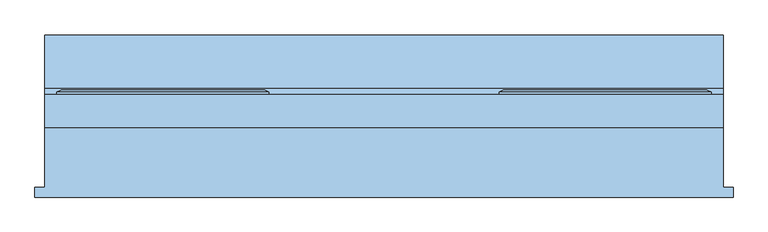
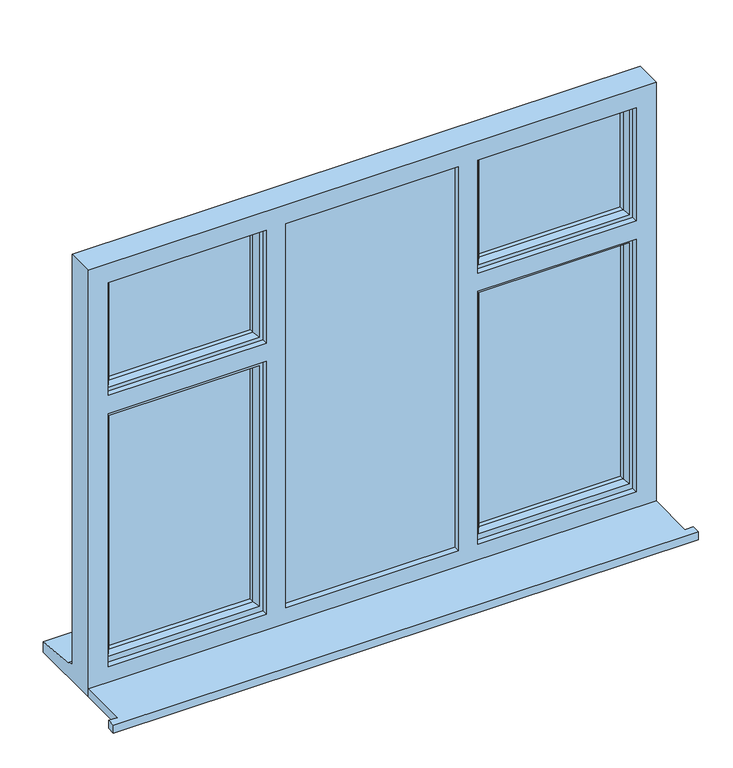
"""IFC4 building model written with IfcOpenShell, lengths in millimetres: window geometry, Window - Triple Casement with Top and Side Sashes : Window - Triple Casement with Top and Side Sashes 1700."""

import ifcopenshell
import ifcopenshell.guid

model = None  # the IFC model being written
_history = None  # IfcOwnerHistory: only IFC2X3 demands one
_inside = {}  # id of a spatial element -> (the spatial element, [elements in it])
_under = {}  # id of a project, library or spatial element -> (it, [spatial elements below it])
_declared = {}  # id of a project -> (the project, [libraries it declares])
_typed = {}  # id of a type object -> (the type object, [elements of that type])
_made_of = {}  # id of a material, layer set ... -> (it, [elements and type objects made of it])


def new_model(schema):
    """Start an empty IFC model of exactly this schema.

    Asked for "IFC4X3", IfcOpenShell would pick the latest addendum, in which some entities
    have other attributes; the version numbers below select the first issue.
    IFC2X3 requires an IfcOwnerHistory on every rooted entity: one is made here for all.
    """
    global model, _history
    if schema == "IFC4X3":
        model = ifcopenshell.file(schema_version=(4, 3, 0, 0))
    else:
        model = ifcopenshell.file(schema=schema)
    _inside.clear()
    _under.clear()
    _declared.clear()
    _typed.clear()
    _made_of.clear()
    _history = None
    if model.schema == "IFC2X3":
        org = make("IfcOrganization", Name="unknown")
        user = make(
            "IfcPersonAndOrganization",
            ThePerson=make("IfcPerson", FamilyName="unknown"),
            TheOrganization=org,
        )
        app = make(
            "IfcApplication",
            ApplicationDeveloper=org,
            Version="unknown",
            ApplicationFullName="unknown",
            ApplicationIdentifier="unknown",
        )
        _history = make(
            "IfcOwnerHistory",
            OwningUser=user,
            OwningApplication=app,
            ChangeAction="ADDED",
            CreationDate=0,
        )
    return model


def make(cls, **values):
    """One entity of the class cls with the attributes given. An attribute that is None is left unset."""
    return model.create_entity(
        cls, **{name: value for name, value in values.items() if value is not None}
    )


def rooted(cls, **values):
    """An entity with a GlobalId (a new one), such as an element, a storey or a relation."""
    return make(cls, GlobalId=ifcopenshell.guid.new(), OwnerHistory=_history, **values)


def si_unit(unit_type, name, prefix=None):
    """IfcSIUnit, for example si_unit("LENGTHUNIT", "METRE", prefix="MILLI")."""
    return make("IfcSIUnit", UnitType=unit_type, Prefix=prefix, Name=name)


def assignment(units):
    """IfcUnitAssignment: the units of a project."""
    return None if units is None else make("IfcUnitAssignment", Units=units)


def point(xyz):
    """IfcCartesianPoint."""
    return None if xyz is None else make("IfcCartesianPoint", Coordinates=xyz)


def direction(xyz):
    """IfcDirection."""
    return None if xyz is None else make("IfcDirection", DirectionRatios=xyz)


def frame(location, z_axis=None, x_axis=None):
    """IfcAxis2Placement3D, a coordinate frame: its origin and axes. An axis left out is left unset."""
    return make(
        "IfcAxis2Placement3D",
        Location=point(location),
        Axis=direction(z_axis),
        RefDirection=direction(x_axis),
    )


def origin():
    """The frame at (0, 0, 0) with its axes left unset."""
    return frame((0.0, 0.0, 0.0))


def place(relative_to, where):
    """IfcLocalPlacement: puts the frame where relative to a parent placement (None: the world)."""
    return make(
        "IfcLocalPlacement", PlacementRelTo=relative_to, RelativePlacement=where
    )


def context(
    kind, dimensions, precision=None, world=None, true_north=None, identifier=None
):
    """IfcGeometricRepresentationContext, for example the 3D "Model" context."""
    return make(
        "IfcGeometricRepresentationContext",
        ContextIdentifier=identifier,
        ContextType=kind,
        CoordinateSpaceDimension=dimensions,
        Precision=precision,
        WorldCoordinateSystem=world,
        TrueNorth=true_north,
    )


def project(units=None, contexts=None):
    """IfcProject with its units and contexts."""
    return rooted(
        "IfcProject",
        Name="project",
        RepresentationContexts=contexts,
        UnitsInContext=assignment(units),
    )


def spatial(cls, under=None, at=None, **own):
    """A site, building, storey or space (cls), placed at a placement, below another one or the project."""
    s = rooted(cls, ObjectPlacement=at, **own)
    if under is not None:
        _under.setdefault(under.id(), (under, []))[1].append(s)
    return s


def polyline(points):
    """IfcPolyline through the points."""
    return make("IfcPolyline", Points=[point(p) for p in points])


def outline(outer, holes=None, kind="AREA"):
    """IfcArbitraryClosedProfileDef: a profile drawn as a closed curve; with holes, ...WithVoids."""
    if holes is None:
        return make("IfcArbitraryClosedProfileDef", ProfileType=kind, OuterCurve=outer)
    return make(
        "IfcArbitraryProfileDefWithVoids",
        ProfileType=kind,
        OuterCurve=outer,
        InnerCurves=holes,
    )


def extrude(swept, where, along, depth):
    """IfcExtrudedAreaSolid: the profile swept, set in the frame where, extruded along a direction by depth."""
    return make(
        "IfcExtrudedAreaSolid",
        SweptArea=swept,
        Position=where,
        ExtrudedDirection=direction(along),
        Depth=depth,
    )


def faces_of(points, faces, orient=None, outer=None):
    """IfcFace entities. A face is a list of loops; a loop is a list of indices into points, from 0.

    orient and outer hold one flag for each loop. By default every Orientation is true, the
    first loop of a face is its IfcFaceOuterBound and the others are IfcFaceBound.
    """
    made = []
    for i, loops in enumerate(faces):
        bounds = []
        for j, loop in enumerate(loops):
            is_outer = j == 0 if outer is None else outer[i][j]
            bounds.append(
                make(
                    "IfcFaceOuterBound" if is_outer else "IfcFaceBound",
                    Bound=make("IfcPolyLoop", Polygon=[points[k] for k in loop]),
                    Orientation=True if orient is None else orient[i][j],
                )
            )
        made.append(make("IfcFace", Bounds=bounds))
    return made


def faceted_brep(points, faces, orient=None, outer=None, voids=None):
    """IfcFacetedBrep: a solid bounded by flat faces; with voids (closed shells), ...WithVoids."""
    shared = [point(p) for p in points]
    hull = make("IfcClosedShell", CfsFaces=faces_of(shared, faces, orient, outer))
    if voids is None:
        return make("IfcFacetedBrep", Outer=hull)
    return make(
        "IfcFacetedBrepWithVoids",
        Outer=hull,
        Voids=[
            make(cls, CfsFaces=faces_of(shared, fs, o, b)) for cls, fs, o, b in voids
        ],
    )


def shape(context_of_items, identifier, shape_type, items):
    """IfcShapeRepresentation: the items that make up one representation, for example the "Body"."""
    return make(
        "IfcShapeRepresentation",
        ContextOfItems=context_of_items,
        RepresentationIdentifier=identifier,
        RepresentationType=shape_type,
        Items=items,
    )


def source(mapping_origin, context_of_items, identifier, shape_type, items):
    """IfcRepresentationMap: a shape defined once, which mapped items show again and again."""
    return make(
        "IfcRepresentationMap",
        MappingOrigin=mapping_origin,
        MappedRepresentation=shape(context_of_items, identifier, shape_type, items),
    )


def transform(
    local_origin,
    x_axis=None,
    y_axis=None,
    z_axis=None,
    scale=None,
    scale2=None,
    scale3=None,
    uniform=True,
):
    """IfcCartesianTransformationOperator3D, or its non-uniform kind. x_axis, y_axis, z_axis: its Axis1, 2, 3."""
    if uniform:
        return make(
            "IfcCartesianTransformationOperator3D",
            Axis1=direction(x_axis),
            Axis2=direction(y_axis),
            LocalOrigin=point(local_origin),
            Scale=scale,
            Axis3=direction(z_axis),
        )
    return make(
        "IfcCartesianTransformationOperator3DnonUniform",
        Axis1=direction(x_axis),
        Axis2=direction(y_axis),
        LocalOrigin=point(local_origin),
        Scale=scale,
        Axis3=direction(z_axis),
        Scale2=scale2,
        Scale3=scale3,
    )


def mapped(mapping_source, mapping_target):
    """IfcMappedItem: shows the shape of a source again, moved by a transform."""
    return make(
        "IfcMappedItem", MappingSource=mapping_source, MappingTarget=mapping_target
    )


def made_of(thing, what):
    """Note that an element or type object is made of a material, layer set ...; save() writes the relation."""
    if what is not None:
        _made_of.setdefault(what.id(), (what, []))[1].append(thing)
    return thing


def element(
    cls,
    number,
    at=None,
    inside=None,
    cuts=None,
    type_object=None,
    material=None,
    context=None,
    identifier="Body",
    shape_type=None,
    held_by="IfcProductDefinitionShape",
    body=None,
    shapes=None,
    **own,
):
    """One element of the class cls, such as IfcWall. Its Tag is "e" and its number.

    at: its placement. inside: the storey or other place that contains it. cuts: it is an
    opening in that element (IfcRelVoidsElement). A single representation is given by context,
    identifier, shape_type and body (its items); several are given by shapes. held_by: the class
    of the entity that holds the representations. save() writes the other relations.
    """
    e = rooted(cls, Tag="e%d" % number, ObjectPlacement=at, **own)
    if body is not None:
        shapes = [shape(context, identifier, shape_type, body)]
    if shapes is not None:
        e.Representation = make(held_by, Representations=shapes)
    if inside is not None:
        _inside.setdefault(inside.id(), (inside, []))[1].append(e)
    if cuts is not None:
        rooted(
            "IfcRelVoidsElement", RelatingBuildingElement=cuts, RelatedOpeningElement=e
        )
    if type_object is not None:
        _typed.setdefault(type_object.id(), (type_object, []))[1].append(e)
    return made_of(e, material)


def aggregate(whole, parts):
    """IfcRelAggregates: a whole, such as a stair, and the parts it consists of."""
    return rooted("IfcRelAggregates", RelatingObject=whole, RelatedObjects=parts)


def save(model, path):
    """Write the relations noted so far, then the file.

    IfcRelAggregates (storeys below a building ...), IfcRelContainedInSpatialStructure (elements
    in a storey), IfcRelDefinesByType, IfcRelAssociatesMaterial and IfcRelDeclares: one each for
    every whole, place, type object, material and project.
    """
    for whole, parts in _under.values():
        aggregate(whole, parts)
    for where, things in _inside.values():
        rooted(
            "IfcRelContainedInSpatialStructure",
            RelatedElements=things,
            RelatingStructure=where,
        )
    for kind, things in _typed.values():
        rooted("IfcRelDefinesByType", RelatedObjects=things, RelatingType=kind)
    for what, things in _made_of.values():
        rooted("IfcRelAssociatesMaterial", RelatedObjects=things, RelatingMaterial=what)
    for by, libraries in _declared.values():
        rooted("IfcRelDeclares", RelatingContext=by, RelatedDefinitions=libraries)
    model.write(path)


def window_acdad559(model_context):
    return source(origin(), model_context, "Body", "SolidModel", [
        extrude(outline(polyline([(-1433.3333333, -182.7934322), (-1433.3333333, -157.7934322), (-1408.3333333, -157.7934322), (-1408.3333333, -8.2934322), (291.6666667, -8.2934322), (291.6666667, -157.7934322), (316.6666667, -157.7934322), (316.6666667, -182.7934322), (-1433.3333333, -182.7934322)])), frame((0.0, 0.0, 760.0), z_axis=(0.0, 0.0, 1.0), x_axis=(1.0, 0.0, 0.0)), (0.0, 0.0, 1.0), 25.0),
        extrude(outline(polyline([(823.0, -826.6666667), (823.0, -290.0), (2070.0, -290.0), (2070.0, -826.6666667), (823.0, -826.6666667)]), holes=[polyline([(2060.0, -816.6666667), (2060.0, -300.0), (833.0, -300.0), (833.0, -816.6666667), (2060.0, -816.6666667)])]), frame((0.0, 33.7065678, 0.0), z_axis=(0.0, 1.0, 0.0), x_axis=(0.0, 0.0, 1.0)), (0.0, 0.0, 1.0), 41.0),
        faceted_brep([(-1378.3333333, 74.7065678, 2080.0), (-1378.3333333, 80.4800705, 2080.0), (-1378.3333333, 80.4800705, 1665.0), (-1378.3333333, 74.7065678, 1665.0), (-1368.3333333, 9.7065678, 2070.0), (-1368.3333333, 74.7065678, 2070.0), (-1368.3333333, 74.7065678, 1675.0), (-1368.3333333, 9.7065678, 1675.0), (-1328.3333333, 24.1994677, 2030.0), (-1338.4813711, 9.7065678, 2040.1480377), (-1338.4813711, 9.7065678, 1704.8519623), (-1328.3333333, 24.1994677, 1715.0), (-1328.3333333, 38.7065678, 2030.0), (-1328.3333333, 38.7065678, 1715.0), (-1338.3333333, 62.7065678, 2040.0), (-1338.3333333, 38.7065678, 2040.0), (-1338.3333333, 38.7065678, 1705.0), (-1338.3333333, 62.7065678, 1705.0), (-1328.3333333, 80.4800705, 2030.0), (-1328.3333333, 62.7065678, 2030.0), (-1328.3333333, 62.7065678, 1715.0), (-1328.3333333, 80.4800705, 1715.0), (-1345.7790881, 86.2535732, 2047.4457548), (-1345.7790881, 86.2535732, 1697.5542452), (-1367.5487236, 86.2535732, 2069.2153903), (-1367.5487236, 86.2535732, 1675.7846097), (-846.6666667, 80.4800705, 1665.0), (-846.6666667, 74.7065678, 1665.0), (-856.6666667, 74.7065678, 1675.0), (-856.6666667, 9.7065678, 1675.0), (-886.5186289, 9.7065678, 1704.8519623), (-896.6666667, 24.1994677, 1715.0), (-896.6666667, 38.7065678, 1715.0), (-886.6666667, 38.7065678, 1705.0), (-886.6666667, 62.7065678, 1705.0), (-896.6666667, 62.7065678, 1715.0), (-896.6666667, 80.4800705, 1715.0), (-879.2209119, 86.2535732, 1697.5542452), (-857.4512764, 86.2535732, 1675.7846097), (-846.6666667, 80.4800705, 2080.0), (-846.6666667, 74.7065678, 2080.0), (-856.6666667, 74.7065678, 2070.0), (-856.6666667, 9.7065678, 2070.0), (-886.5186289, 9.7065678, 2040.1480377), (-896.6666667, 24.1994677, 2030.0), (-896.6666667, 38.7065678, 2030.0), (-886.6666667, 38.7065678, 2040.0), (-886.6666667, 62.7065678, 2040.0), (-896.6666667, 62.7065678, 2030.0), (-896.6666667, 80.4800705, 2030.0), (-879.2209119, 86.2535732, 2047.4457548), (-857.4512764, 86.2535732, 2069.2153903)], [[[0, 1, 2, 3]], [[4, 5, 6, 7]], [[8, 9, 10, 11]], [[12, 8, 11, 13]], [[14, 15, 16, 17]], [[18, 19, 20, 21]], [[22, 18, 21, 23]], [[1, 24, 25, 2]], [[3, 2, 26, 27]], [[7, 6, 28, 29]], [[11, 10, 30, 31]], [[13, 11, 31, 32]], [[17, 16, 33, 34]], [[21, 20, 35, 36]], [[23, 21, 36, 37]], [[2, 25, 38, 26]], [[27, 26, 39, 40]], [[29, 28, 41, 42]], [[31, 30, 43, 44]], [[32, 31, 44, 45]], [[34, 33, 46, 47]], [[36, 35, 48, 49]], [[37, 36, 49, 50]], [[26, 38, 51, 39]], [[40, 39, 1, 0]], [[3, 27, 40, 0], [5, 41, 28, 6]], [[42, 41, 5, 4]], [[7, 29, 42, 4], [9, 43, 30, 10]], [[44, 43, 9, 8]], [[45, 44, 8, 12]], [[15, 46, 33, 16], [13, 32, 45, 12]], [[47, 46, 15, 14]], [[17, 34, 47, 14], [19, 48, 35, 20]], [[49, 48, 19, 18]], [[50, 49, 18, 22]], [[24, 51, 38, 25], [23, 37, 50, 22]], [[39, 51, 24, 1]]]),
        faceted_brep([(-1378.3333333, 74.7065678, 1655.0), (-1378.3333333, 80.4800705, 1655.0), (-1378.3333333, 80.4800705, 813.0), (-1378.3333333, 74.7065678, 813.0), (-1368.3333333, 9.7065678, 1645.0), (-1368.3333333, 74.7065678, 1645.0), (-1368.3333333, 74.7065678, 823.0), (-1368.3333333, 9.7065678, 823.0), (-1328.3333333, 24.1994677, 1605.0), (-1338.4813711, 9.7065678, 1615.1480377), (-1338.4813711, 9.7065678, 852.8519623), (-1328.3333333, 24.1994677, 863.0), (-1328.3333333, 38.7065678, 1605.0), (-1328.3333333, 38.7065678, 863.0), (-1338.3333333, 62.7065678, 1615.0), (-1338.3333333, 38.7065678, 1615.0), (-1338.3333333, 38.7065678, 853.0), (-1338.3333333, 62.7065678, 853.0), (-1328.3333333, 80.4800705, 1605.0), (-1328.3333333, 62.7065678, 1605.0), (-1328.3333333, 62.7065678, 863.0), (-1328.3333333, 80.4800705, 863.0), (-1345.7790881, 86.2535732, 1622.4457548), (-1345.7790881, 86.2535732, 845.5542452), (-1367.5487236, 86.2535732, 1644.2153903), (-1367.5487236, 86.2535732, 823.7846097), (-846.6666667, 80.4800705, 813.0), (-846.6666667, 74.7065678, 813.0), (-856.6666667, 74.7065678, 823.0), (-856.6666667, 9.7065678, 823.0), (-886.5186289, 9.7065678, 852.8519623), (-896.6666667, 24.1994677, 863.0), (-896.6666667, 38.7065678, 863.0), (-886.6666667, 38.7065678, 853.0), (-886.6666667, 62.7065678, 853.0), (-896.6666667, 62.7065678, 863.0), (-896.6666667, 80.4800705, 863.0), (-879.2209119, 86.2535732, 845.5542452), (-857.4512764, 86.2535732, 823.7846097), (-846.6666667, 80.4800705, 1655.0), (-846.6666667, 74.7065678, 1655.0), (-856.6666667, 74.7065678, 1645.0), (-856.6666667, 9.7065678, 1645.0), (-886.5186289, 9.7065678, 1615.1480377), (-896.6666667, 24.1994677, 1605.0), (-896.6666667, 38.7065678, 1605.0), (-886.6666667, 38.7065678, 1615.0), (-886.6666667, 62.7065678, 1615.0), (-896.6666667, 62.7065678, 1605.0), (-896.6666667, 80.4800705, 1605.0), (-879.2209119, 86.2535732, 1622.4457548), (-857.4512764, 86.2535732, 1644.2153903)], [[[0, 1, 2, 3]], [[4, 5, 6, 7]], [[8, 9, 10, 11]], [[12, 8, 11, 13]], [[14, 15, 16, 17]], [[18, 19, 20, 21]], [[22, 18, 21, 23]], [[1, 24, 25, 2]], [[3, 2, 26, 27]], [[7, 6, 28, 29]], [[11, 10, 30, 31]], [[13, 11, 31, 32]], [[17, 16, 33, 34]], [[21, 20, 35, 36]], [[23, 21, 36, 37]], [[2, 25, 38, 26]], [[27, 26, 39, 40]], [[29, 28, 41, 42]], [[31, 30, 43, 44]], [[32, 31, 44, 45]], [[34, 33, 46, 47]], [[36, 35, 48, 49]], [[37, 36, 49, 50]], [[26, 38, 51, 39]], [[40, 39, 1, 0]], [[3, 27, 40, 0], [5, 41, 28, 6]], [[42, 41, 5, 4]], [[7, 29, 42, 4], [9, 43, 30, 10]], [[44, 43, 9, 8]], [[45, 44, 8, 12]], [[15, 46, 33, 16], [13, 32, 45, 12]], [[47, 46, 15, 14]], [[17, 34, 47, 14], [19, 48, 35, 20]], [[49, 48, 19, 18]], [[50, 49, 18, 22]], [[24, 51, 38, 25], [23, 37, 50, 22]], [[39, 51, 24, 1]]]),
        faceted_brep([(-270.0, 74.7065678, 2080.0), (-270.0, 80.4800705, 2080.0), (-270.0, 80.4800705, 1665.0), (-270.0, 74.7065678, 1665.0), (-260.0, 9.7065678, 2070.0), (-260.0, 74.7065678, 2070.0), (-260.0, 74.7065678, 1675.0), (-260.0, 9.7065678, 1675.0), (-220.0, 24.1994677, 2030.0), (-230.1480377, 9.7065678, 2040.1480377), (-230.1480377, 9.7065678, 1704.8519623), (-220.0, 24.1994677, 1715.0), (-220.0, 38.7065678, 2030.0), (-220.0, 38.7065678, 1715.0), (-230.0, 62.7065678, 2040.0), (-230.0, 38.7065678, 2040.0), (-230.0, 38.7065678, 1705.0), (-230.0, 62.7065678, 1705.0), (-220.0, 80.4800705, 2030.0), (-220.0, 62.7065678, 2030.0), (-220.0, 62.7065678, 1715.0), (-220.0, 80.4800705, 1715.0), (-237.4457548, 86.2535732, 2047.4457548), (-237.4457548, 86.2535732, 1697.5542452), (-259.2153903, 86.2535732, 2069.2153903), (-259.2153903, 86.2535732, 1675.7846097), (261.6666667, 80.4800705, 1665.0), (261.6666667, 74.7065678, 1665.0), (251.6666667, 74.7065678, 1675.0), (251.6666667, 9.7065678, 1675.0), (221.8147044, 9.7065678, 1704.8519623), (211.6666667, 24.1994677, 1715.0), (211.6666667, 38.7065678, 1715.0), (221.6666667, 38.7065678, 1705.0), (221.6666667, 62.7065678, 1705.0), (211.6666667, 62.7065678, 1715.0), (211.6666667, 80.4800705, 1715.0), (229.1124215, 86.2535732, 1697.5542452), (250.882057, 86.2535732, 1675.7846097), (261.6666667, 80.4800705, 2080.0), (261.6666667, 74.7065678, 2080.0), (251.6666667, 74.7065678, 2070.0), (251.6666667, 9.7065678, 2070.0), (221.8147044, 9.7065678, 2040.1480377), (211.6666667, 24.1994677, 2030.0), (211.6666667, 38.7065678, 2030.0), (221.6666667, 38.7065678, 2040.0), (221.6666667, 62.7065678, 2040.0), (211.6666667, 62.7065678, 2030.0), (211.6666667, 80.4800705, 2030.0), (229.1124215, 86.2535732, 2047.4457548), (250.882057, 86.2535732, 2069.2153903)], [[[0, 1, 2, 3]], [[4, 5, 6, 7]], [[8, 9, 10, 11]], [[12, 8, 11, 13]], [[14, 15, 16, 17]], [[18, 19, 20, 21]], [[22, 18, 21, 23]], [[1, 24, 25, 2]], [[3, 2, 26, 27]], [[7, 6, 28, 29]], [[11, 10, 30, 31]], [[13, 11, 31, 32]], [[17, 16, 33, 34]], [[21, 20, 35, 36]], [[23, 21, 36, 37]], [[2, 25, 38, 26]], [[27, 26, 39, 40]], [[29, 28, 41, 42]], [[31, 30, 43, 44]], [[32, 31, 44, 45]], [[34, 33, 46, 47]], [[36, 35, 48, 49]], [[37, 36, 49, 50]], [[26, 38, 51, 39]], [[40, 39, 1, 0]], [[3, 27, 40, 0], [5, 41, 28, 6]], [[42, 41, 5, 4]], [[7, 29, 42, 4], [9, 43, 30, 10]], [[44, 43, 9, 8]], [[45, 44, 8, 12]], [[15, 46, 33, 16], [13, 32, 45, 12]], [[47, 46, 15, 14]], [[17, 34, 47, 14], [19, 48, 35, 20]], [[49, 48, 19, 18]], [[50, 49, 18, 22]], [[24, 51, 38, 25], [23, 37, 50, 22]], [[39, 51, 24, 1]]]),
        extrude(outline(polyline([(221.6666667, 38.7065678), (-230.1480377, 38.7065678), (-230.1480377, 62.7065678), (221.6666667, 62.7065678), (221.6666667, 38.7065678)])), frame((0.0, 0.0, 852.8519623), z_axis=(0.0, 0.0, 1.0), x_axis=(1.0, 0.0, 0.0)), (0.0, 0.0, 1.0), 762.1480377),
        extrude(outline(polyline([(221.6666667, 38.7065678), (-230.0, 38.7065678), (-230.0, 62.7065678), (221.6666667, 62.7065678), (221.6666667, 38.7065678)])), frame((0.0, 0.0, 1705.0), z_axis=(0.0, 0.0, 1.0), x_axis=(1.0, 0.0, 0.0)), (0.0, 0.0, 1.0), 335.0),
        extrude(outline(polyline([(-886.6666667, 38.7065678), (-1338.3333333, 38.7065678), (-1338.3333333, 62.7065678), (-886.6666667, 62.7065678), (-886.6666667, 38.7065678)])), frame((0.0, 0.0, 1705.0), z_axis=(0.0, 0.0, 1.0), x_axis=(1.0, 0.0, 0.0)), (0.0, 0.0, 1.0), 335.0),
        extrude(outline(polyline([(-886.6666667, 38.7065678), (-1338.3333333, 38.7065678), (-1338.3333333, 62.7065678), (-886.6666667, 62.7065678), (-886.6666667, 38.7065678)])), frame((0.0, 0.0, 853.0), z_axis=(0.0, 0.0, 1.0), x_axis=(1.0, 0.0, 0.0)), (0.0, 0.0, 1.0), 762.0),
        faceted_brep([(-270.0, 74.7065678, 1655.0), (-270.0, 80.4800705, 1655.0), (-270.0, 80.4800705, 813.0), (-270.0, 74.7065678, 813.0), (-260.0, 9.7065678, 1645.0), (-260.0, 74.7065678, 1645.0), (-260.0, 74.7065678, 823.0), (-260.0, 9.7065678, 823.0), (-220.0, 24.1994677, 1605.0), (-230.1480377, 9.7065678, 1615.1480377), (-230.1480377, 9.7065678, 852.8519623), (-220.0, 24.1994677, 863.0), (-220.0, 38.7065678, 1605.0), (-220.0, 38.7065678, 863.0), (-230.0, 62.7065678, 1615.0), (-230.0, 38.7065678, 1615.0), (-230.0, 38.7065678, 853.0), (-230.0, 62.7065678, 853.0), (-220.0, 80.4800705, 1605.0), (-220.0, 62.7065678, 1605.0), (-220.0, 62.7065678, 863.0), (-220.0, 80.4800705, 863.0), (-237.4457548, 86.2535732, 1622.4457548), (-237.4457548, 86.2535732, 845.5542452), (-259.2153903, 86.2535732, 1644.2153903), (-259.2153903, 86.2535732, 823.7846097), (261.6666667, 80.4800705, 813.0), (261.6666667, 74.7065678, 813.0), (251.6666667, 74.7065678, 823.0), (251.6666667, 9.7065678, 823.0), (221.8147044, 9.7065678, 852.8519623), (211.6666667, 24.1994677, 863.0), (211.6666667, 38.7065678, 863.0), (221.6666667, 38.7065678, 853.0), (221.6666667, 62.7065678, 853.0), (211.6666667, 62.7065678, 863.0), (211.6666667, 80.4800705, 863.0), (229.1124215, 86.2535732, 845.5542452), (250.882057, 86.2535732, 823.7846097), (261.6666667, 80.4800705, 1655.0), (261.6666667, 74.7065678, 1655.0), (251.6666667, 74.7065678, 1645.0), (251.6666667, 9.7065678, 1645.0), (221.8147044, 9.7065678, 1615.1480377), (211.6666667, 24.1994677, 1605.0), (211.6666667, 38.7065678, 1605.0), (221.6666667, 38.7065678, 1615.0), (221.6666667, 62.7065678, 1615.0), (211.6666667, 62.7065678, 1605.0), (211.6666667, 80.4800705, 1605.0), (229.1124215, 86.2535732, 1622.4457548), (250.882057, 86.2535732, 1644.2153903)], [[[0, 1, 2, 3]], [[4, 5, 6, 7]], [[8, 9, 10, 11]], [[12, 8, 11, 13]], [[14, 15, 16, 17]], [[18, 19, 20, 21]], [[22, 18, 21, 23]], [[1, 24, 25, 2]], [[3, 2, 26, 27]], [[7, 6, 28, 29]], [[11, 10, 30, 31]], [[13, 11, 31, 32]], [[17, 16, 33, 34]], [[21, 20, 35, 36]], [[23, 21, 36, 37]], [[2, 25, 38, 26]], [[27, 26, 39, 40]], [[29, 28, 41, 42]], [[31, 30, 43, 44]], [[32, 31, 44, 45]], [[34, 33, 46, 47]], [[36, 35, 48, 49]], [[37, 36, 49, 50]], [[26, 38, 51, 39]], [[40, 39, 1, 0]], [[3, 27, 40, 0], [5, 41, 28, 6]], [[42, 41, 5, 4]], [[7, 29, 42, 4], [9, 43, 30, 10]], [[44, 43, 9, 8]], [[45, 44, 8, 12]], [[15, 46, 33, 16], [13, 32, 45, 12]], [[47, 46, 15, 14]], [[17, 34, 47, 14], [19, 48, 35, 20]], [[49, 48, 19, 18]], [[50, 49, 18, 22]], [[24, 51, 38, 25], [23, 37, 50, 22]], [[39, 51, 24, 1]]]),
        faceted_brep([(291.6666667, -8.2934322, 2110.0), (-1408.3333333, -8.2934322, 2110.0), (-1408.3333333, -8.2934322, 760.0), (291.6666667, -8.2934322, 760.0), (231.6666667, -8.2934322, 835.0), (-242.0, -8.2934322, 835.0), (-242.0, -8.2934322, 1635.0), (231.6666667, -8.2934322, 1635.0), (-816.6666667, -8.2934322, 2050.0), (-300.0, -8.2934322, 2050.0), (-300.0, -8.2934322, 835.0), (-816.6666667, -8.2934322, 835.0), (-242.0, -8.2934322, 2050.0), (231.6666667, -8.2934322, 2050.0), (231.6666667, -8.2934322, 1693.0), (-242.0, -8.2934322, 1693.0), (-1348.3333333, -8.2934322, 835.0), (-1348.3333333, -8.2934322, 1635.0), (-874.6666667, -8.2934322, 1635.0), (-874.6666667, -8.2934322, 835.0), (-1348.3333333, -8.2934322, 2050.0), (-874.6666667, -8.2934322, 2050.0), (-874.6666667, -8.2934322, 1693.0), (-1348.3333333, -8.2934322, 1693.0), (-1408.3333333, 74.7065678, 2110.0), (-1408.3333333, 74.7065678, 811.0), (-1408.3333333, 89.7065678, 809.68767), (-1408.3333333, 89.7065678, 804.7449676), (-1408.3333333, 224.7065678, 793.8088847), (-1408.3333333, 224.7065678, 760.0), (291.6666667, 74.7065678, 2110.0), (291.6666667, 74.7065678, 811.0), (-260.0, 74.7065678, 823.0), (251.6666667, 74.7065678, 823.0), (251.6666667, 74.7065678, 1645.0), (-260.0, 74.7065678, 1645.0), (251.6666667, 74.7065678, 2070.0), (-260.0, 74.7065678, 2070.0), (-260.0, 74.7065678, 1675.0), (251.6666667, 74.7065678, 1675.0), (-856.6666667, 74.7065678, 823.0), (-856.6666667, 74.7065678, 1645.0), (-1368.3333333, 74.7065678, 1645.0), (-1368.3333333, 74.7065678, 823.0), (-856.6666667, 74.7065678, 2070.0), (-1368.3333333, 74.7065678, 2070.0), (-1368.3333333, 74.7065678, 1675.0), (-856.6666667, 74.7065678, 1675.0), (-816.6666667, 74.7065678, 2070.0), (-816.6666667, 74.7065678, 823.0), (-300.0, 74.7065678, 823.0), (-300.0, 74.7065678, 2070.0), (-1368.3333333, 9.7065678, 2070.0), (-1368.3333333, 9.7065678, 1675.0), (-1368.3333333, 9.7065678, 1645.0), (-1368.3333333, 9.7065678, 823.0), (-856.6666667, 9.7065678, 2070.0), (-856.6666667, 9.7065678, 1675.0), (-874.6666667, 9.7065678, 2050.0), (-1348.3333333, 9.7065678, 2050.0), (-1348.3333333, 9.7065678, 1693.0), (-874.6666667, 9.7065678, 1693.0), (-260.0, 9.7065678, 2070.0), (251.6666667, 9.7065678, 2070.0), (251.6666667, 9.7065678, 1675.0), (-260.0, 9.7065678, 1675.0), (231.6666667, 9.7065678, 2050.0), (-242.0, 9.7065678, 2050.0), (-242.0, 9.7065678, 1693.0), (231.6666667, 9.7065678, 1693.0), (-826.6666667, 9.7065678, 2070.0), (-290.0, 9.7065678, 2070.0), (-290.0, 9.7065678, 823.0), (-826.6666667, 9.7065678, 823.0), (-300.0, 9.7065678, 2050.0), (-816.6666667, 9.7065678, 2050.0), (-816.6666667, 9.7065678, 835.0), (-300.0, 9.7065678, 835.0), (-856.6666667, 9.7065678, 823.0), (-856.6666667, 9.7065678, 1645.0), (-1348.3333333, 9.7065678, 835.0), (-874.6666667, 9.7065678, 835.0), (-874.6666667, 9.7065678, 1635.0), (-1348.3333333, 9.7065678, 1635.0), (251.6666667, 9.7065678, 823.0), (-260.0, 9.7065678, 823.0), (-260.0, 9.7065678, 1645.0), (251.6666667, 9.7065678, 1645.0), (-242.0, 9.7065678, 835.0), (231.6666667, 9.7065678, 835.0), (231.6666667, 9.7065678, 1635.0), (-242.0, 9.7065678, 1635.0), (-816.6666667, 33.7065678, 2070.0), (-300.0, 33.7065678, 2070.0), (-290.0, 33.7065678, 2070.0), (-826.6666667, 33.7065678, 2070.0), (291.6666667, 224.7065678, 760.0), (291.6666667, 224.7065678, 793.8088847), (291.6666667, 89.7065678, 804.7449676), (291.6666667, 89.7065678, 809.68767), (-816.6666667, 33.7065678, 823.0), (-826.6666667, 33.7065678, 823.0), (-290.0, 33.7065678, 823.0), (-300.0, 33.7065678, 823.0)], [[[0, 1, 2, 3], [4, 5, 6, 7], [8, 9, 10, 11], [12, 13, 14, 15], [16, 17, 18, 19], [20, 21, 22, 23]], [[1, 24, 25, 26, 27, 28, 29, 2]], [[24, 30, 31, 25], [32, 33, 34, 35], [36, 37, 38, 39], [40, 41, 42, 43], [44, 45, 46, 47], [48, 49, 50, 51]], [[45, 52, 53, 46]], [[54, 55, 43, 42]], [[52, 56, 57, 53], [58, 59, 60, 61]], [[62, 63, 64, 65], [66, 67, 68, 69]], [[70, 71, 72, 73], [74, 75, 76, 77]], [[78, 55, 54, 79], [80, 81, 82, 83]], [[84, 85, 86, 87], [88, 89, 90, 91]], [[59, 20, 23, 60]], [[16, 80, 83, 17]], [[1, 0, 30, 24]], [[52, 45, 44, 56]], [[36, 63, 62, 37]], [[92, 48, 51, 93, 94, 71, 70, 95]], [[20, 59, 58, 21]], [[66, 13, 12, 67]], [[8, 75, 74, 9]], [[30, 0, 3, 96, 97, 98, 99, 31]], [[63, 36, 39, 64]], [[33, 84, 87, 34]], [[13, 66, 69, 14]], [[89, 4, 7, 90]], [[75, 8, 11, 76]], [[21, 58, 61, 22]], [[81, 19, 18, 82]], [[57, 56, 44, 47]], [[40, 78, 79, 41]], [[49, 48, 92, 100]], [[100, 92, 95, 101]], [[101, 95, 70, 73]], [[94, 102, 72, 71]], [[102, 94, 93, 103]], [[103, 93, 51, 50]], [[37, 62, 65, 38]], [[85, 32, 35, 86]], [[67, 12, 15, 68]], [[5, 88, 91, 6]], [[9, 74, 77, 10]], [[96, 3, 2, 29]], [[97, 96, 29, 28]], [[98, 97, 28, 27]], [[99, 98, 27, 26]], [[31, 99, 26, 25]], [[33, 32, 85, 84]], [[40, 43, 55, 78]], [[50, 49, 100, 101, 73, 72, 102, 103]], [[5, 4, 89, 88]], [[77, 76, 11, 10]], [[81, 80, 16, 19]], [[35, 34, 87, 86]], [[39, 38, 65, 64]], [[15, 14, 69, 68]], [[7, 6, 91, 90]], [[47, 46, 53, 57]], [[42, 41, 79, 54]], [[83, 82, 18, 17]], [[61, 60, 23, 22]]]),
        extrude(outline(polyline([(-826.6666667, 33.7065678), (-290.0, 33.7065678), (-290.0, 9.7065678), (-826.6666667, 9.7065678), (-826.6666667, 33.7065678)])), frame((0.0, 0.0, 823.0), z_axis=(0.0, 0.0, 1.0), x_axis=(1.0, 0.0, 0.0)), (0.0, 0.0, 1.0), 1247.0),
    ])


if __name__ == "__main__":
    model = new_model("IFC4")
    model_context = context("Model", 3, world=origin())
    ifc_project = project(units=[si_unit("LENGTHUNIT", "METRE", prefix="MILLI")], contexts=[model_context])
    site = spatial("IfcSite", under=ifc_project)
    building = spatial("IfcBuilding", under=site)
    placement = place(None, origin())
    window_shape = window_acdad559(model_context)
    element("IfcWindow", 1, ObjectType="Window - Triple Casement with Top and Side Sashes : Window - Triple Casement with Top and Side Sashes 1700", at=placement, inside=building, context=model_context, shape_type="MappedRepresentation", body=[
        mapped(window_shape, transform((0.0, 0.0, 0.0), x_axis=(1.0, 0.0, 0.0), y_axis=(0.0, 1.0, 0.0), z_axis=(0.0, 0.0, 1.0))),
    ])
    save(model, "model.ifc")

# Revit data of these elements
# Project information
#   Document_Suitability_Code = "A1"
#   Document_Suitability_Description = "Coordination"
#   Project Status = "Project Status"
#   Client Name = "Revit Project"
#   Project Address = "Enter address here"
#   Project Name = "Two Storey Residence"
#   Project Number = "RARC01"
# Type "Window - Triple Casement with Top and Side Sashes : Window - Triple Casement with Top and Side Sashes 1700"
#   Description = "Triple Casement Window with Opening Sash Vents"
#   Type Mark = "60"
#   Operation = "Userdefined"
#   Manufacturer = "Revit"
#   Keynote = "L10"
#   Wrap Layers (Ext) from Ext = 100 mm
#   Wrap Layers (Int) from Ext = 177.5 mm
#   Window Board Projection = 25 mm
#   Window Board Extension = 25 mm
#   Visual Light Transmittance = 0.9
#   Vent Height = 450 mm
#   Solar Heat Gain Coefficient = 0.78
#   Rough Width = 1700 mm
#   Rough Height = 1350 mm
#   Height = 1350 mm
#   Width = 1700 mm
#   Heat Transfer Coefficient (U) = 3.6886 W/(m²·K)
#   Glazing Thickness = 24 mm
#   FrameOffset - External = 100 mm
#   Frame Depth = 65 mm
#   Default Head Height = 2110 mm
#   Cill Depth = 150 mm
#   Cavity Closer Width = 50 mm
#   Cavity Closer Offset from Ext = 102.5 mm
#   Cavity Closer Depth = 85 mm
#   Vis - Cavity Closers = yes
#   Define Thermal Properties by = 1
#   Material Trim = Window Frame
#   Material Glass = Glass
#   Material Frame = Window Frame
#   Construction Type Id = ""
#   Wall Closure = (empty or 0)
#   Analytic Construction = (empty or 0)
# Element 1 (IfcWindow, "Window - Triple Casement with Top and Side Sashes : Window - Triple Casement with Top and Side Sashes 1700")
#   Materials on its faces: "Window Frame", "Glass"
# Materials
#   "Window Frame": class "Miscellaneous", colour RGB 249 249 249, transparency 0, Keynote = "L10"
#   "Glass": class "Glass", colour RGB 0 128 192, transparency 0.9, Description = "Soda Lime Glass", Cost = 0
